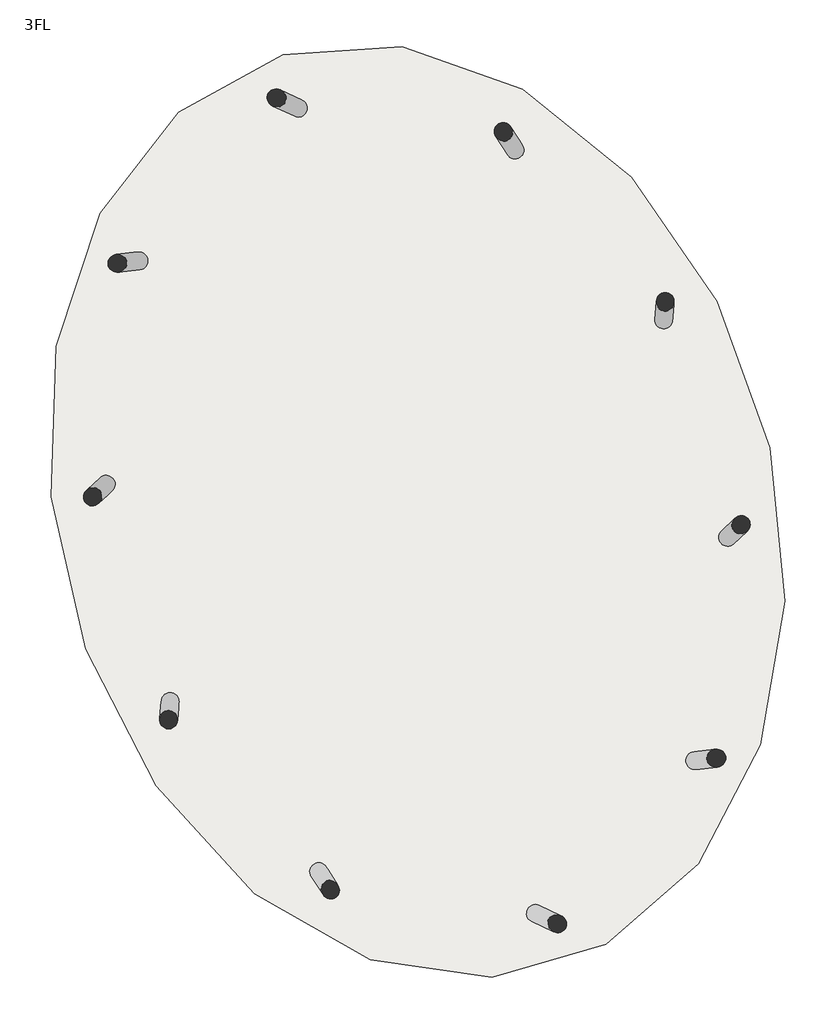
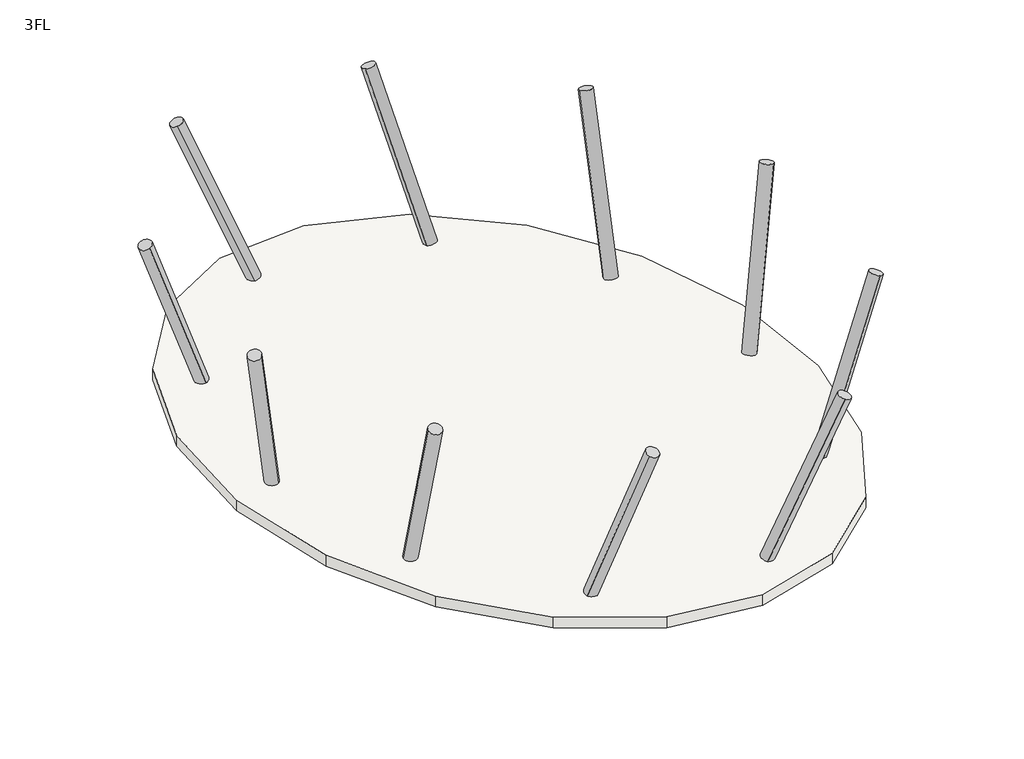
# One storey: 10 columns, 1 slab.
"""IFC4 building model written with IfcOpenShell, lengths in millimetres."""

from ifc_helpers import new_model, si_unit, point, frame, frame_2d, origin, place, context, project, spatial, polyline, circle_curve, trimmed, segment, composite_curve, outline, extrude, element, save

model = new_model("IFC4")

# Units and contexts
model_context = context("Model", 3, world=origin())
ifc_project = project(units=[si_unit("LENGTHUNIT", "METRE", prefix="MILLI")], contexts=[model_context])

# Site, building, storey
site = spatial("IfcSite", under=ifc_project)
building = spatial("IfcBuilding", under=site)
storey = spatial("IfcBuildingStorey", under=building, Name="3FL", Elevation=9000.0)

# Columns
placement = place(None, origin())
element("IfcColumn", 1, ObjectType="コンクリート-円形-柱 : 750", at=placement, inside=storey, context=model_context, shape_type="SweptSolid", body=[
    extrude(outline(composite_curve([segment(trimmed(circle_curve(frame_2d((0.0, -175.0)), 175.0), [point((0.0, -350.0))], [point((0.0, 0.0))], False, "CARTESIAN"), True, "CONTINUOUS"), segment(trimmed(circle_curve(frame_2d((0.0, -175.0)), 175.0), [point((0.0, 0.0))], [point((0.0, -350.0))], False, "CARTESIAN"), True, "CONTINUOUS")], self_intersect=False)), frame((-2396.4430027, 7751.2725912, 9000.0), z_axis=(-0.33782365532567055, 0.15733612172811007, 0.9279657982393317), x_axis=(-0.8412072169935014, 0.391779199013945, -0.3726653690618973)), (0.0, 0.0, 1.0), 4849.3166543),
])
element("IfcColumn", 2, ObjectType="コンクリート-円形-柱 : 750", at=placement, inside=storey, context=model_context, shape_type="SweptSolid", body=[
    extrude(outline(composite_curve([segment(trimmed(circle_curve(frame_2d((0.0, -174.9999999)), 175.0), [point((0.0, -350.0))], [point((0.0, 0.0))], False, "CARTESIAN"), True, "CONTINUOUS"), segment(trimmed(circle_curve(frame_2d((0.0, -174.9999999)), 175.0), [point((0.0, 0.0))], [point((0.0, -350.0))], False, "CARTESIAN"), True, "CONTINUOUS")], self_intersect=False)), frame((-5437.5169545, 4739.0498309, 9000.0), z_axis=(-0.3386274608575676, -0.03887699204723502, 0.9401170258231236), x_axis=(-0.9339818734574898, -0.10722817864420414, -0.3408518413585062)), (0.0, 0.0, 1.0), 4786.6381274),
])
element("IfcColumn", 3, ObjectType="コンクリート-円形-柱 : 750", at=placement, inside=storey, context=model_context, shape_type="SweptSolid", body=[
    extrude(outline(composite_curve([segment(trimmed(circle_curve(frame_2d((0.0, -175.0)), 175.0), [point((0.0, -350.0))], [point((0.0, 0.0))], False, "CARTESIAN"), True, "CONTINUOUS"), segment(trimmed(circle_curve(frame_2d((0.0, -175.0)), 175.0), [point((0.0, 0.0))], [point((0.0, -350.0))], False, "CARTESIAN"), True, "CONTINUOUS")], self_intersect=False)), frame((-5986.4478133, 398.1248489, 9000.0), z_axis=(-0.21390210927369444, -0.1995400513533381, 0.9562581531961816), x_axis=(-0.699243725622998, -0.6522943106689199, -0.292524092077607)), (0.0, 0.0, 1.0), 4705.8422299),
])
element("IfcColumn", 4, ObjectType="コンクリート-円形-柱 : 750", at=placement, inside=storey, context=model_context, shape_type="SweptSolid", body=[
    extrude(outline(composite_curve([segment(trimmed(circle_curve(frame_2d((0.0, -175.0)), 175.0), [point((0.0, -350.0))], [point((0.0, 0.0))], False, "CARTESIAN"), True, "CONTINUOUS"), segment(trimmed(circle_curve(frame_2d((0.0, -175.0)), 175.0), [point((0.0, 0.0))], [point((0.0, -350.0))], False, "CARTESIAN"), True, "CONTINUOUS")], self_intersect=False)), frame((-4677.7670005, -3758.6917761, 9000.0), z_axis=(-0.02500202504056698, -0.28943616606306627, 0.9568707355325401), x_axis=(-0.0823495752042211, -0.9533205924463546, -0.2905140194231872)), (0.0, 0.0, 1.0), 4702.8295826),
])
element("IfcColumn", 5, ObjectType="コンクリート-円形-柱 : 750", at=placement, inside=storey, context=model_context, shape_type="SweptSolid", body=[
    extrude(outline(composite_curve([segment(trimmed(circle_curve(frame_2d((-1e-07, -175.0000001)), 175.0), [point((0.0, -350.0000001))], [point((0.0, 0.0))], False, "CARTESIAN"), True, "CONTINUOUS"), segment(trimmed(circle_curve(frame_2d((-1e-07, -175.0000001)), 175.0), [point((0.0, 0.0))], [point((0.0, -350.0000001))], False, "CARTESIAN"), True, "CONTINUOUS")], self_intersect=False)), frame((-1787.6399598, -6989.1483955, 9000.0), z_axis=(0.1823560991835319, -0.28470523350892224, 0.9411106115134372), x_axis=(0.5075949581961906, -0.7924875655283201, -0.3380988271153925)), (0.0, 0.0, 1.0), 4781.5845864),
])
element("IfcColumn", 6, ObjectType="コンクリート-円形-柱 : 750", at=placement, inside=storey, context=model_context, shape_type="SweptSolid", body=[
    extrude(outline(composite_curve([segment(trimmed(circle_curve(frame_2d((0.0, -175.0)), 175.0), [point((0.0, -350.0))], [point((0.0, 0.0))], False, "CARTESIAN"), True, "CONTINUOUS"), segment(trimmed(circle_curve(frame_2d((0.0, -175.0)), 175.0), [point((0.0, 0.0))], [point((0.0, -350.0))], False, "CARTESIAN"), True, "CONTINUOUS")], self_intersect=False)), frame((2396.4430382, -7751.2725943, 9000.0), z_axis=(0.3378236555427887, -0.15733612109966955, 0.9279657982668421), x_axis=(0.8412072177137112, -0.3917791975327104, -0.3726653689933942)), (0.0, 0.0, 1.0), 4849.3166543),
])
element("IfcColumn", 7, ObjectType="コンクリート-円形-柱 : 750", at=placement, inside=storey, context=model_context, shape_type="SweptSolid", body=[
    extrude(outline(composite_curve([segment(trimmed(circle_curve(frame_2d((-1e-07, -175.0)), 175.0), [point((-1e-07, -350.0))], [point((0.0, 0.0))], False, "CARTESIAN"), True, "CONTINUOUS"), segment(trimmed(circle_curve(frame_2d((-1e-07, -175.0)), 175.0), [point((0.0, 0.0))], [point((-1e-07, -350.0))], False, "CARTESIAN"), True, "CONTINUOUS")], self_intersect=False)), frame((5437.5169384, -4739.0497953, 9000.0), z_axis=(0.33862746188616666, 0.03887699356383296, 0.9401170253899089), x_axis=(0.9339818725900185, 0.10722818240188961, -0.34085184255337325)), (0.0, 0.0, 1.0), 4786.6381274),
])
element("IfcColumn", 8, ObjectType="コンクリート-円形-柱 : 750", at=placement, inside=storey, context=model_context, shape_type="SweptSolid", body=[
    extrude(outline(composite_curve([segment(trimmed(circle_curve(frame_2d((0.0, -175.0000001)), 175.0), [point((0.0, -350.0))], [point((0.0, 0.0))], False, "CARTESIAN"), True, "CONTINUOUS"), segment(trimmed(circle_curve(frame_2d((0.0, -175.0000001)), 175.0), [point((0.0, 0.0))], [point((0.0, -350.0))], False, "CARTESIAN"), True, "CONTINUOUS")], self_intersect=False)), frame((5986.4477911, -398.1248264, 9000.0), z_axis=(0.21390210829237388, 0.1995400534687371, 0.9562581529742746), x_axis=(0.699243720518798, 0.6522943158151849, -0.2925240928030184)), (0.0, 0.0, 1.0), 4705.8422299),
])
element("IfcColumn", 9, ObjectType="コンクリート-円形-柱 : 750", at=placement, inside=storey, context=model_context, shape_type="SweptSolid", body=[
    extrude(outline(composite_curve([segment(trimmed(circle_curve(frame_2d((-1e-07, -175.0)), 175.0), [point((0.0, -350.0))], [point((0.0, 0.0))], False, "CARTESIAN"), True, "CONTINUOUS"), segment(trimmed(circle_curve(frame_2d((-1e-07, -175.0)), 175.0), [point((0.0, 0.0))], [point((0.0, -350.0))], False, "CARTESIAN"), True, "CONTINUOUS")], self_intersect=False)), frame((4677.7669981, 3758.6917817, 9000.0), z_axis=(0.025002026568373387, 0.28943616430058094, 0.95687073602574), x_axis=(0.08234958073929972, 0.9533205924632611, -0.2905140177987261)), (0.0, 0.0, 1.0), 4702.8295826),
])
element("IfcColumn", 10, ObjectType="コンクリート-円形-柱 : 750", at=placement, inside=storey, context=model_context, shape_type="SweptSolid", body=[
    extrude(outline(composite_curve([segment(trimmed(circle_curve(frame_2d((0.0, -175.0000001)), 175.0), [point((0.0, -350.0000001))], [point((0.0, 0.0))], False, "CARTESIAN"), True, "CONTINUOUS"), segment(trimmed(circle_curve(frame_2d((0.0, -175.0000001)), 175.0), [point((0.0, 0.0))], [point((0.0, -350.0000001))], False, "CARTESIAN"), True, "CONTINUOUS")], self_intersect=False)), frame((1787.6399702, 6989.1484212, 9000.0), z_axis=(-0.18235609571736613, 0.28470523085765614, 0.9411106129871278), x_axis=(-0.5075949555013638, 0.7924875690044456, -0.3380988230133203)), (0.0, 0.0, 1.0), 4781.5845864),
])

# Slab
element("IfcSlab", 11, ObjectType="一般 300 mm", at=placement, inside=storey, context=model_context, shape_type="SweptSolid", body=[
    extrude(outline(polyline([(-6230.4914027, 5847.2181447), (-4689.4663855, 7832.2134964), (-2633.1542325, 8967.6997676), (-289.3841433, 9124.1942139), (2080.1781062, 8287.4508866), (4218.6193751, 6554.8946324), (5898.8223826, 4116.9204503), (6942.687748, 1236.3865471), (7238.7435529, -1777.7303478), (6753.8172257, -4602.436936), (5536.3004014, -6933.8710897), (3712.7542311, -8516.7556068), (1481.138097, -9172.0172073), (-908.6985378, -8826.2935355), (-3193.4073344, -7523.2055995), (-5128.5050121, -5409.0821813), (-6509.001626, -2713.3858267), (-7188.1804107, 274.2297181), (-7092.7720452, 3233.5704394), (-6230.4914027, 5847.2181447)])), frame((0.0, 0.0, 8700.0), z_axis=(0.0, 0.0, 1.0), x_axis=(1.0, 0.0, 0.0)), (0.0, 0.0, 1.0), 300.0),
])

save(model, "model.ifc")

# Revit data of these elements
# Type "コンクリート-円形-柱 : 750"
#   Keynote = "03310.Q1"
#   R = 350 mm
#   Structural Material [instance default] = コンクリート - 現場打ち
# Type "一般 300 mm"
#   Function = 0
#   Layers, outside or top first: 300 mm no material (function 1)
# Elements 1, 2, 3, 4, 5, 6, 7, 8, 9, 10 (IfcColumn, "コンクリート-円形-柱 : 750")
#   Structural Material = コンクリート - 現場打ち
#   Phase Created = 新しい建設
#   Materials on its faces: "コンクリート - 現場打ち"
# Element 11 (IfcSlab, "一般 300 mm")
#   Height Offset From Level = 0 mm
#   Phase Created = 新しい建設
# Materials
#   "コンクリート - 現場打ち": class "コンクリート", colour RGB 192 192 192, transparency 0
